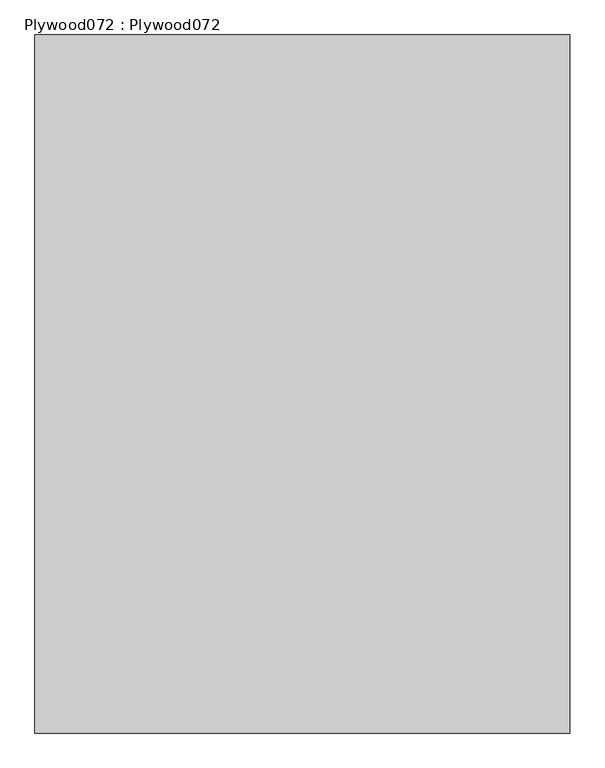
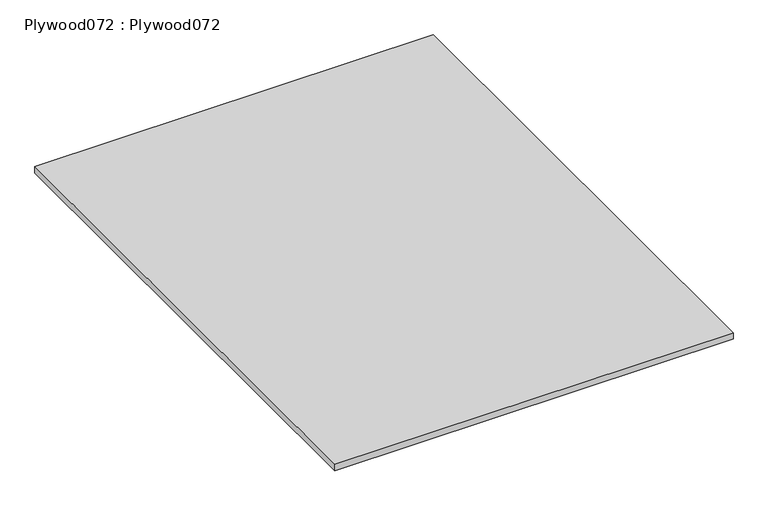
"""IFC4 building model written with IfcOpenShell, lengths in millimetres: proxy geometry, Plywood072 : Plywood072."""

from ifc_helpers import new_model, si_unit, frame, origin, place, context, project, spatial, polyline, outline, extrude, source, transform, mapped, element, save


def plywood072_plywood072_49e20a31(model_context):
    return source(origin(), model_context, "Body", "SweptSolid", [
        extrude(outline(polyline([(-4952.2707965, 7982.1531721), (-6484.1211227, 7982.1531721), (-6484.1211227, 9982.1531721), (-4952.2707965, 9982.1531721), (-4952.2707965, 7982.1531721)])), frame((0.0, 0.0, 43411.8082994), z_axis=(0.0, 0.0, 1.0), x_axis=(1.0, 0.0, 0.0)), (0.0, 0.0, 1.0), 26.0465759),
    ])


if __name__ == "__main__":
    model = new_model("IFC4")
    model_context = context("Model", 3, world=origin())
    ifc_project = project(units=[si_unit("LENGTHUNIT", "METRE", prefix="MILLI")], contexts=[model_context])
    site = spatial("IfcSite", under=ifc_project)
    building = spatial("IfcBuilding", under=site)
    placement = place(None, origin())
    plywood072_plywood072_shape = plywood072_plywood072_49e20a31(model_context)
    element("IfcBuildingElementProxy", 1, Name="Plywood072 : Plywood072", ObjectType="Plywood072 : Plywood072", at=placement, inside=building, context=model_context, shape_type="MappedRepresentation", body=[
        mapped(plywood072_plywood072_shape, transform((0.0, 0.0, 0.0), x_axis=(1.0, 0.0, 0.0), y_axis=(0.0, 1.0, 0.0), z_axis=(0.0, 0.0, 1.0))),
    ])
    save(model, "model.ifc")

# Revit data of these elements
# Type "Plywood072 : Plywood072"
#   NameOverride = "Plywood072"
# Element 1 (IfcBuildingElementProxy, "Plywood072 : Plywood072")
#   Materials on its faces: "CDX PLYWOOD - SEE STRUCTURAL DWGS"
# Materials
#   "CDX PLYWOOD - SEE STRUCTURAL DWGS": class "Unassigned", colour RGB 177 130 114, transparency 0, Cost = 0
